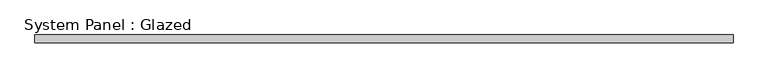
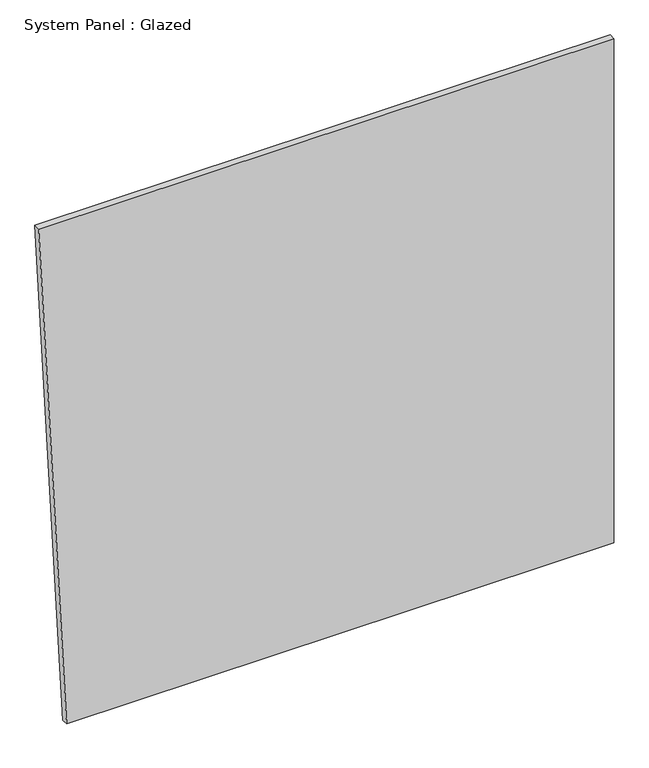
"""IFC4 building model written with IfcOpenShell, lengths in millimetres: plate geometry, System Panel : Glazed."""

from ifc_helpers import new_model, si_unit, frame, origin, place, context, project, spatial, polyline, outline, extrude, source, transform, mapped, element, save


def system_panel_glazed_282f07fc(model_context):
    return source(origin(), model_context, "Body", "SweptSolid", [
        extrude(outline(polyline([(0.0, -1017.0034845), (0.0, 1126.1853377), (2086.1728929, 1126.1853377), (2086.1728929, -1126.1853377), (0.0, -1017.0034845)])), frame((0.0, -44.45, 0.0), z_axis=(0.0, 1.0, 0.0), x_axis=(0.0, 0.0, 1.0)), (0.0, 0.0, 1.0), 25.4),
    ])


if __name__ == "__main__":
    model = new_model("IFC4")
    model_context = context("Model", 3, world=origin())
    ifc_project = project(units=[si_unit("LENGTHUNIT", "METRE", prefix="MILLI")], contexts=[model_context])
    site = spatial("IfcSite", under=ifc_project)
    building = spatial("IfcBuilding", under=site)
    placement = place(None, origin())
    system_panel_glazed_shape = system_panel_glazed_282f07fc(model_context)
    element("IfcPlate", 1, ObjectType="System Panel : Glazed", at=placement, inside=building, context=model_context, shape_type="MappedRepresentation", body=[
        mapped(system_panel_glazed_shape, transform((0.0, 0.0, 0.0), x_axis=(1.0, 0.0, 0.0), y_axis=(0.0, 1.0, 0.0), z_axis=(0.0, 0.0, 1.0))),
    ])
    save(model, "model.ifc")

# Revit data of these elements
# Type "System Panel : Glazed"
#   Construction Type Id = "GSP4R"
#   Analytic Construction = "1/8 in Pilkington single glazing"
#   Visual Light Transmittance = 0.9
#   Solar Heat Gain Coefficient = 0.86
#   Heat Transfer Coefficient (U) = 1.18115 BTU/(h·ft²·°F)
#   Define Thermal Properties by = 1
# Element 1 (IfcPlate, "System Panel : Glazed")
#   Materials on its faces: "Glass"
# Materials
#   "Glass": class "Glass", colour RGB 0 128 192, transparency 0.75, Description = "Soda Lime Glass", Cost = 0
